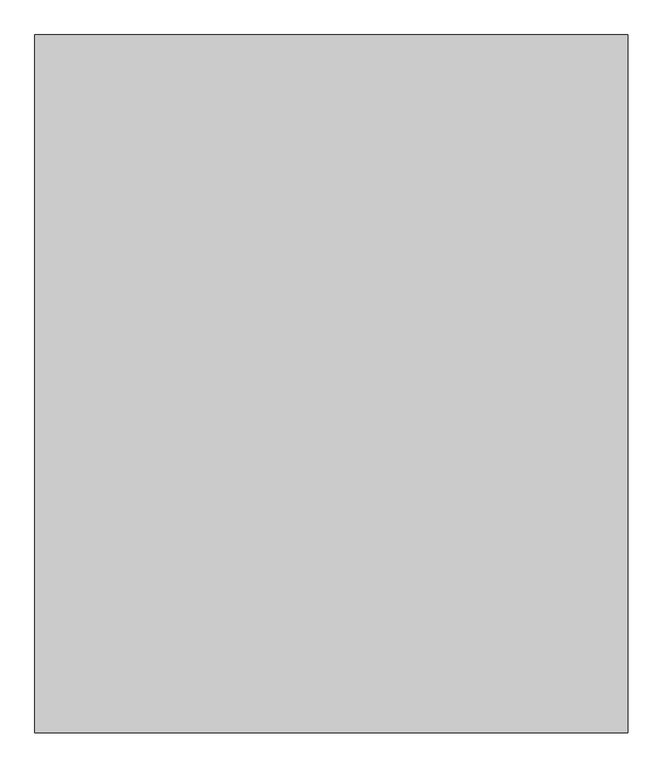
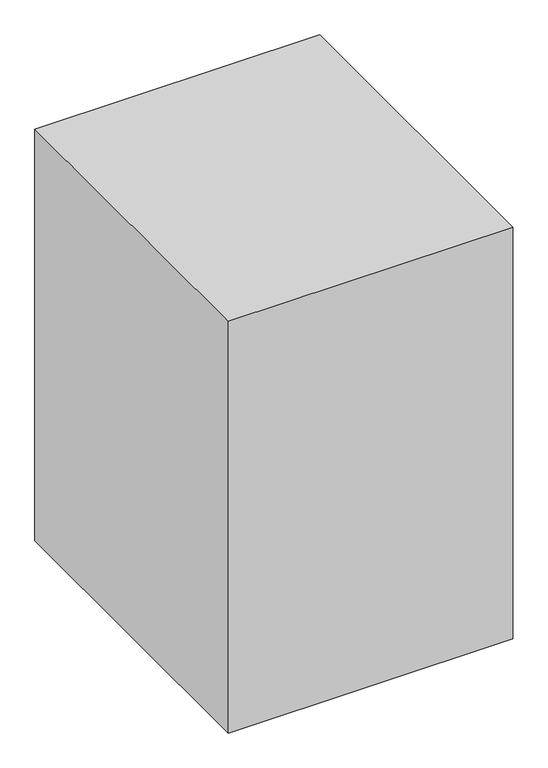
"""IFC4 building model written with IfcOpenShell, lengths in millimetres: proxy geometry, Space Planning Box_hec : Space Planning Box_hec."""

from ifc_helpers import new_model, si_unit, origin, origin_with_axes, place, context, project, spatial, polyline, outline, extrude, source, transform, mapped, element, save


def generic_models_5d679b5e(model_context):
    return source(origin(), model_context, "Body", "SweptSolid", [
        extrude(outline(polyline([(1700.0, 2000.0), (1700.0, -2000.0), (-1700.0, -2000.0), (-1700.0, 2000.0), (1700.0, 2000.0)])), origin_with_axes(), (0.0, 0.0, 1.0), 5200.0),
    ])


if __name__ == "__main__":
    model = new_model("IFC4")
    model_context = context("Model", 3, world=origin())
    ifc_project = project(units=[si_unit("LENGTHUNIT", "METRE", prefix="MILLI")], contexts=[model_context])
    site = spatial("IfcSite", under=ifc_project)
    building = spatial("IfcBuilding", under=site)
    placement = place(None, origin())
    generic_models_shape = generic_models_5d679b5e(model_context)
    element("IfcBuildingElementProxy", 1, Name="Space Planning Box_hec : Space Planning Box_hec", ObjectType="Space Planning Box_hec : Space Planning Box_hec", at=placement, inside=building, context=model_context, shape_type="MappedRepresentation", body=[
        mapped(generic_models_shape, transform((0.0, 0.0, 0.0), x_axis=(1.0, 0.0, 0.0), y_axis=(0.0, 1.0, 0.0), z_axis=(0.0, 0.0, 1.0))),
    ])
    save(model, "model.ifc")

# Revit data of these elements
# Type "Space Planning Box_hec : Space Planning Box_hec"
#   Type Comments = "..."
#   Room Name [instance default] = "?"
#   Interior Finish [instance default] = ""
#   Exterior Finish [instance default] = ""
#   Department [instance default] = ""
#   Assembly Code = "..."
#   ceiling height [instance default] = 0
#   Width [instance default] = 1524 mm
#   Program Area [instance default] = 0.00 m²
#   Length [instance default] = 1524 mm
#   Height [instance default] = 1524 mm
#   Area [instance default] = 2.32258 m²
#   Fill Color [instance default] = Cyan
#   Default Elevation = 0
# Element 1 (IfcBuildingElementProxy, "Space Planning Box_hec : Space Planning Box_hec")
#   Room Name = "Toilet(F)"
#   Interior Finish = "IW3..N/A,,N/A..N/A,,FL5..N/A,,CL5..N/A"
#   Exterior Finish = "N/A..N/A,,EW1..N/A"
#   Department = "AR"
#   ceiling height = 2400
#   Width = 3400 mm
#   Program Area = 13.60 m²
#   Length = 4000 mm
#   Height = 5200 mm
#   Area = 13.60 m²
#   Materials on its faces: "Cyan"
# Materials
#   "Cyan": class "Generic", colour RGB 0 255 255, transparency 0.2, Cost = 0
